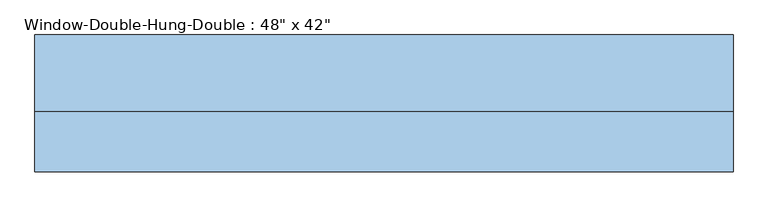
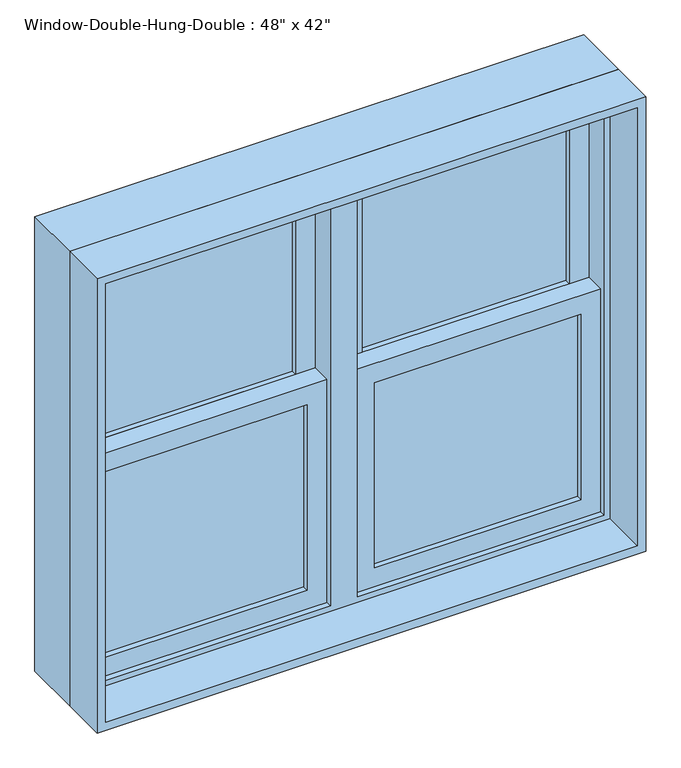
"""IFC4 building model written with IfcOpenShell, lengths in millimetres: window geometry."""

from ifc_helpers import new_model, si_unit, frame, origin, place, context, project, spatial, polyline, outline, extrude, source, transform, mapped, element, save


def window_9e3aa26a(model_context):
    return source(origin(), model_context, "Body", "SweptSolid", [
        extrude(outline(polyline([(1981.2, 609.6), (1981.2, -609.6), (914.4, -609.6), (914.4, 609.6), (1981.2, 609.6)]), holes=[polyline([(946.15, -577.85), (1949.45, -577.85), (1949.45, -30.1625), (946.15, -30.1625), (946.15, -577.85)]), polyline([(946.15, 577.85), (946.15, 30.1625), (1949.45, 30.1625), (1949.45, 577.85), (946.15, 577.85)])]), frame((0.0, -4.3, 0.0), z_axis=(0.0, 1.0, 0.0), x_axis=(0.0, 0.0, 1.0)), (0.0, 0.0, 1.0), 133.35),
        extrude(outline(polyline([(-533.4, 40.15), (-74.6125, 40.15), (-74.6125, 33.8), (-533.4, 33.8), (-533.4, 40.15)])), frame((0.0, 0.0, 990.6), z_axis=(0.0, 0.0, 1.0), x_axis=(1.0, 0.0, 0.0)), (0.0, 0.0, 1.0), 434.975),
        extrude(outline(polyline([(-74.6125, 27.45), (-74.6125, 21.1), (-533.4, 21.1), (-533.4, 27.45), (-74.6125, 27.45)])), frame((0.0, 0.0, 990.6), z_axis=(0.0, 0.0, 1.0), x_axis=(1.0, 0.0, 0.0)), (0.0, 0.0, 1.0), 434.975),
        extrude(outline(polyline([(-533.4, 84.6), (-74.6125, 84.6), (-74.6125, 78.25), (-533.4, 78.25), (-533.4, 84.6)])), frame((0.0, 0.0, 1470.025), z_axis=(0.0, 0.0, 1.0), x_axis=(1.0, 0.0, 0.0)), (0.0, 0.0, 1.0), 434.975),
        extrude(outline(polyline([(-74.6125, 71.9), (-74.6125, 65.55), (-533.4, 65.55), (-533.4, 71.9), (-74.6125, 71.9)])), frame((0.0, 0.0, 1470.025), z_axis=(0.0, 0.0, 1.0), x_axis=(1.0, 0.0, 0.0)), (0.0, 0.0, 1.0), 434.975),
        extrude(outline(polyline([(1470.025, -577.85), (946.15, -577.85), (946.15, -30.1625), (1470.025, -30.1625), (1470.025, -577.85)]), holes=[polyline([(1425.575, -74.6125), (990.6, -74.6125), (990.6, -533.4), (1425.575, -533.4), (1425.575, -74.6125)])]), frame((0.0, 8.4, 0.0), z_axis=(0.0, 1.0, 0.0), x_axis=(0.0, 0.0, 1.0)), (0.0, 0.0, 1.0), 44.45),
        extrude(outline(polyline([(1949.45, -577.85), (1425.575, -577.85), (1425.575, -30.1625), (1949.45, -30.1625), (1949.45, -577.85)]), holes=[polyline([(1905.0, -74.6125), (1470.025, -74.6125), (1470.025, -533.4), (1905.0, -533.4), (1905.0, -74.6125)])]), frame((0.0, 52.85, 0.0), z_axis=(0.0, 1.0, 0.0), x_axis=(0.0, 0.0, 1.0)), (0.0, 0.0, 1.0), 44.45),
        extrude(outline(polyline([(533.4, 40.15), (533.4, 33.8), (74.6125, 33.8), (74.6125, 40.15), (533.4, 40.15)])), frame((0.0, 0.0, 990.6), z_axis=(0.0, 0.0, 1.0), x_axis=(1.0, 0.0, 0.0)), (0.0, 0.0, 1.0), 434.975),
        extrude(outline(polyline([(74.6125, 27.45), (533.4, 27.45), (533.4, 21.1), (74.6125, 21.1), (74.6125, 27.45)])), frame((0.0, 0.0, 990.6), z_axis=(0.0, 0.0, 1.0), x_axis=(1.0, 0.0, 0.0)), (0.0, 0.0, 1.0), 434.975),
        extrude(outline(polyline([(533.4, 84.6), (533.4, 78.25), (74.6125, 78.25), (74.6125, 84.6), (533.4, 84.6)])), frame((0.0, 0.0, 1470.025), z_axis=(0.0, 0.0, 1.0), x_axis=(1.0, 0.0, 0.0)), (0.0, 0.0, 1.0), 434.975),
        extrude(outline(polyline([(74.6125, 71.9), (533.4, 71.9), (533.4, 65.55), (74.6125, 65.55), (74.6125, 71.9)])), frame((0.0, 0.0, 1470.025), z_axis=(0.0, 0.0, 1.0), x_axis=(1.0, 0.0, 0.0)), (0.0, 0.0, 1.0), 434.975),
        extrude(outline(polyline([(1470.025, 30.1625), (946.15, 30.1625), (946.15, 577.85), (1470.025, 577.85), (1470.025, 30.1625)]), holes=[polyline([(1425.575, 533.4), (990.6, 533.4), (990.6, 74.6125), (1425.575, 74.6125), (1425.575, 533.4)])]), frame((0.0, 8.4, 0.0), z_axis=(0.0, 1.0, 0.0), x_axis=(0.0, 0.0, 1.0)), (0.0, 0.0, 1.0), 44.45),
        extrude(outline(polyline([(1949.45, 30.1625), (1425.575, 30.1625), (1425.575, 577.85), (1949.45, 577.85), (1949.45, 30.1625)]), holes=[polyline([(1905.0, 533.4), (1470.025, 533.4), (1470.025, 74.6125), (1905.0, 74.6125), (1905.0, 533.4)])]), frame((0.0, 52.85, 0.0), z_axis=(0.0, 1.0, 0.0), x_axis=(0.0, 0.0, 1.0)), (0.0, 0.0, 1.0), 44.45),
        extrude(outline(polyline([(1981.2, 609.6), (1981.2, -609.6), (914.4, -609.6), (914.4, 609.6), (1981.2, 609.6)]), holes=[polyline([(1962.15, 590.55), (933.45, 590.55), (933.45, -590.55), (1962.15, -590.55), (1962.15, 590.55)])]), frame((0.0, -110.0, 0.0), z_axis=(0.0, 1.0, 0.0), x_axis=(0.0, 0.0, 1.0)), (0.0, 0.0, 1.0), 105.7),
    ])


if __name__ == "__main__":
    model = new_model("IFC4")
    model_context = context("Model", 3, world=origin())
    ifc_project = project(units=[si_unit("LENGTHUNIT", "METRE", prefix="MILLI")], contexts=[model_context])
    site = spatial("IfcSite", under=ifc_project)
    building = spatial("IfcBuilding", under=site)
    placement = place(None, origin())
    window_shape = window_9e3aa26a(model_context)
    element("IfcWindow", 1, ObjectType="Window-Double-Hung-Double : 48\" x 42\"", at=placement, inside=building, context=model_context, shape_type="MappedRepresentation", body=[
        mapped(window_shape, transform((0.0, 0.0, 0.0), x_axis=(1.0, 0.0, 0.0), y_axis=(0.0, 1.0, 0.0), z_axis=(0.0, 0.0, 1.0))),
    ])
    save(model, "model.ifc")

# Revit data of these elements
# Type "Window-Double-Hung-Double : 48\" x 42\""
#   Type Mark = "32"
#   Fire Rating = "0.5h"
#   Construction Type Id = "DG-DR"
#   Assembly Code = "B2020100"
#   Analytic Construction = "Double glazing - domestic"
#   Wall Thickness [instance default] = 15.24 cm
#   Window Inset [instance default] = 0 cm
#   Visual Light Transmittance = 0.81
#   Thermal Resistance (R) = 0.319569 (m²·K)/W
#   Solar Heat Gain Coefficient = 0.76
#   Muntin Width = 45.8787 cm
#   Muntin Height = 43.4975 cm
#   Interior Wall Closure [instance default] = 3.81 cm
#   Rough Width = 123.19 cm
#   Rough Height = 107.95 cm
#   Frame Extension [instance default] = 3.175 cm
#   Exterior Wall Closure [instance default] = 1.27 cm
#   Extension Jamb [instance default] = 3.81 cm
#   Heat Transfer Coefficient (U) = 3.12929 W/(m²·K)
#   Height = 106.68 cm
#   Width = 121.92 cm
#   Top Muntin Visibility = yes
#   Indicator Visibility [instance default] = yes
#   Extension Jamb Visibility [instance default] = yes
#   Interior Trim Visibility [instance default] = yes
#   Exterior Trim Visibility [instance default] = yes
#   Bottom Muntin Visibility = yes
#   Muntin Pattern = Muntin Pattern_2x2 : Muntin Pattern_2x2
#   Interior Trim Material = Wood - Stained
#   Interior Trim = Trim-Window-Interior-Flat : Picture Frame
#   Exterior Trim Material = Clad - White
#   Exterior Trim = Trim-Window-Exterior-Flat : with Sill
#   Glass Panel Material = Glass
#   Exterior Frame Material = Clad - White
#   Interior Frame Material = Wood - Stained
#   Wall Closure = (empty or 0)
# Element 1 (IfcWindow, "Window-Double-Hung-Double : 48\" x 42\"")
#   Wall Thickness = 22 cm
#   Extension Jamb = 10.57 cm
#   Materials on its faces: "Wood - Stained", "Glass", "Clad - White"
# Materials
#   "Wood - Stained": class "Wood", colour RGB 224 178 126, transparency 0, Cost = 0
#   "Clad - White": class "Wood", colour RGB 242 242 238, transparency 0, Cost = 0
#   "Glass": class "Glass", colour RGB 0 128 192, transparency 0.9, Description = "Soda Lime Glass", Cost = 0
